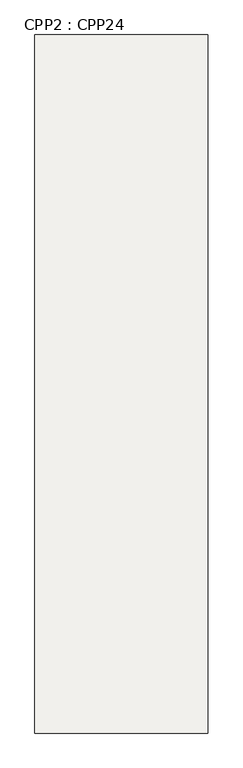
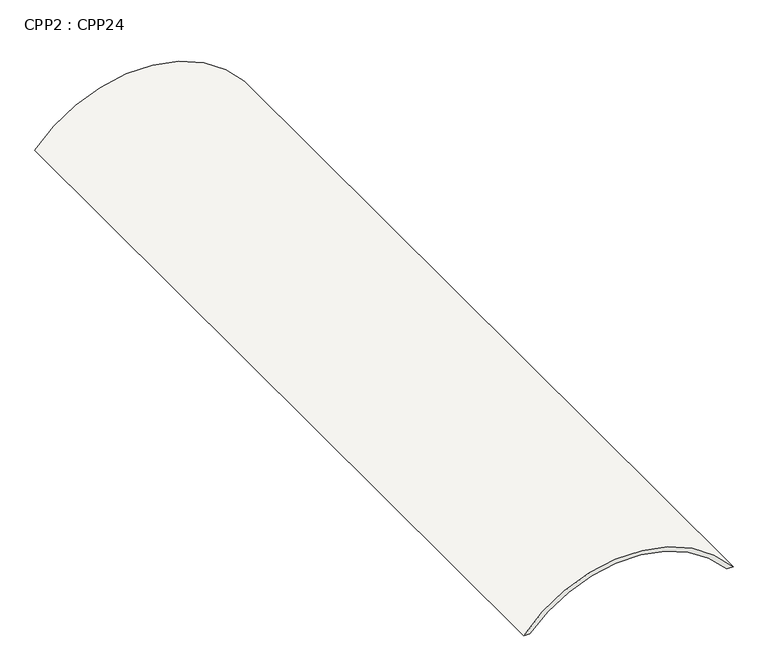
"""IFC4 building model written with IfcOpenShell, lengths in millimetres: slab geometry, CPP2 : CPP24."""

from ifc_helpers import new_model, si_unit, point, frame, frame_2d, origin, place, context, project, spatial, polyline, circle_curve, trimmed, segment, composite_curve, outline, extrude, source, transform, mapped, element, save


def cpp2_cpp24_ee28efaa(model_context):
    return source(origin(), model_context, "Body", "SweptSolid", [
        extrude(outline(composite_curve([segment(polyline([(14620.0, 30333.2245515), (14620.0, 30483.2245515)]), True, "CONTINUOUS"), segment(trimmed(circle_curve(frame_2d((12603.2870371, 32833.2245514)), 3096.7129629), [point((14620.0, 30483.2245515))], [point((14620.0, 35183.2245514))], True, "CARTESIAN"), True, "CONTINUOUS"), segment(polyline([(14620.0, 35183.2245514), (14620.0, 35333.2245514)]), True, "CONTINUOUS"), segment(trimmed(circle_curve(frame_2d((12561.6949153, 32833.2245514)), 3238.3050847), [point((14620.0, 35333.2245514))], [point((14620.0, 30333.2245515))], False, "CARTESIAN"), True, "CONTINUOUS")], self_intersect=False)), frame((0.0, -100.2551788, 0.0), z_axis=(0.0, 1.0, 0.0), x_axis=(0.0, 0.0, 1.0)), (0.0, 0.0, 1.0), 20199.9999981),
    ])


if __name__ == "__main__":
    model = new_model("IFC4")
    model_context = context("Model", 3, world=origin())
    ifc_project = project(units=[si_unit("LENGTHUNIT", "METRE", prefix="MILLI")], contexts=[model_context])
    site = spatial("IfcSite", under=ifc_project)
    building = spatial("IfcBuilding", under=site)
    placement = place(None, origin())
    cpp2_cpp24_shape = cpp2_cpp24_ee28efaa(model_context)
    element("IfcSlab", 1, ObjectType="CPP2 : CPP24", at=placement, inside=building, context=model_context, shape_type="MappedRepresentation", body=[
        mapped(cpp2_cpp24_shape, transform((0.0, 0.0, 0.0), x_axis=(1.0, 0.0, 0.0), y_axis=(0.0, 1.0, 0.0), z_axis=(0.0, 0.0, 1.0))),
    ])
    save(model, "model.ifc")

# Revit data of these elements
# Element 1 (IfcSlab, "CPP2 : CPP24")
#   Materials on its faces: "Concrete, RC"
# Materials
#   "Concrete, RC": class "Concrete", colour RGB 128 128 128, transparency 0, Description = "Cast-in-place concrete", Cost = 0
